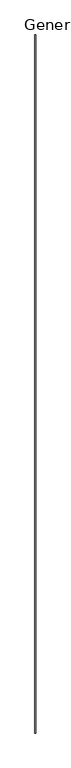
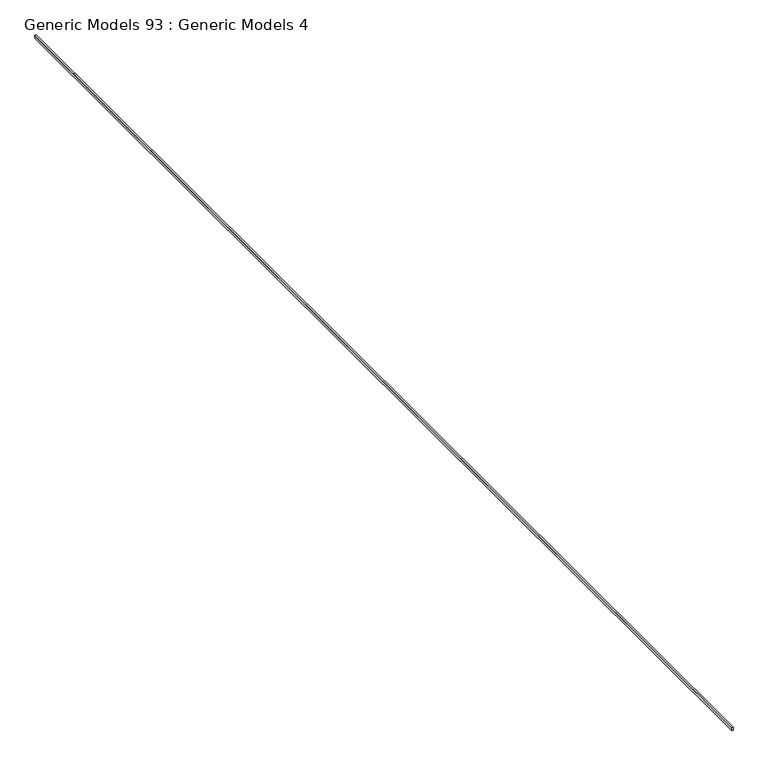
"""IFC4 building model written with IfcOpenShell, lengths in millimetres: proxy geometry, Generic Models 93 : Generic Models 4."""

from ifc_helpers import new_model, si_unit, frame, origin, place, context, project, spatial, polyline, outline, extrude, source, transform, mapped, element, save


def generic_models_93_generic_models_4_66edce56(model_context):
    return source(origin(), model_context, "Body", "SweptSolid", [
        extrude(outline(polyline([(126305.691, -9003.6381655), (126357.126, -9003.6381655), (126357.126, -9020.6881401), (126353.6462, -9020.6881401), (126353.6462, -9021.9581401), (126305.691, -9021.9581401), (126305.691, -9003.6381655)])), frame((0.0, -6864.9230338, 0.0), z_axis=(0.0, 1.0, 0.0), x_axis=(0.0, 0.0, 1.0)), (0.0, 0.0, 1.0), 18643.6),
    ])


if __name__ == "__main__":
    model = new_model("IFC4")
    model_context = context("Model", 3, world=origin())
    ifc_project = project(units=[si_unit("LENGTHUNIT", "METRE", prefix="MILLI")], contexts=[model_context])
    site = spatial("IfcSite", under=ifc_project)
    building = spatial("IfcBuilding", under=site)
    placement = place(None, origin())
    generic_models_93_generic_models_4_shape = generic_models_93_generic_models_4_66edce56(model_context)
    element("IfcBuildingElementProxy", 1, Name="Generic Models 93 : Generic Models 4", ObjectType="Generic Models 93 : Generic Models 4", at=placement, inside=building, context=model_context, shape_type="MappedRepresentation", body=[
        mapped(generic_models_93_generic_models_4_shape, transform((0.0, 0.0, 0.0), x_axis=(1.0, 0.0, 0.0), y_axis=(0.0, 1.0, 0.0), z_axis=(0.0, 0.0, 1.0))),
    ])
    save(model, "model.ifc")

# Revit data of these elements
# Element 1 (IfcBuildingElementProxy, "Generic Models 93 : Generic Models 4")
#   Materials on its faces: "_7/8\" SMOOTH TROWEL EXTERIOR STUCCO (COLOR PER OWNER)"
# Materials
#   "_7/8\" SMOOTH TROWEL EXTERIOR STUCCO (COLOR PER OWNER)": class "Generic", colour RGB 233 233 233, transparency 0, Cost = 0
